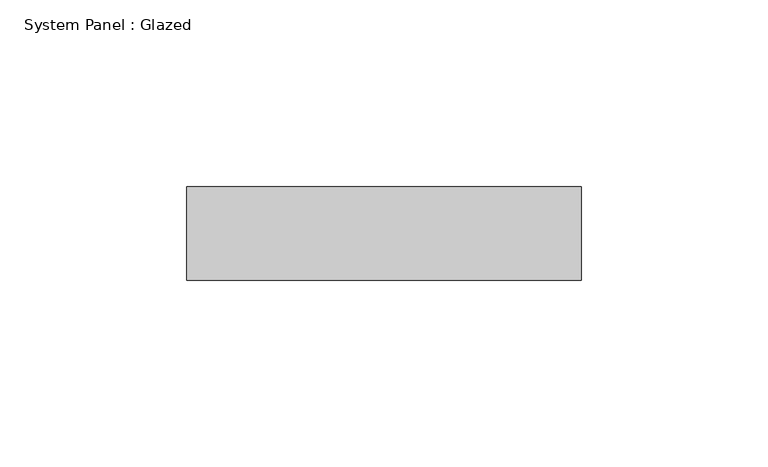
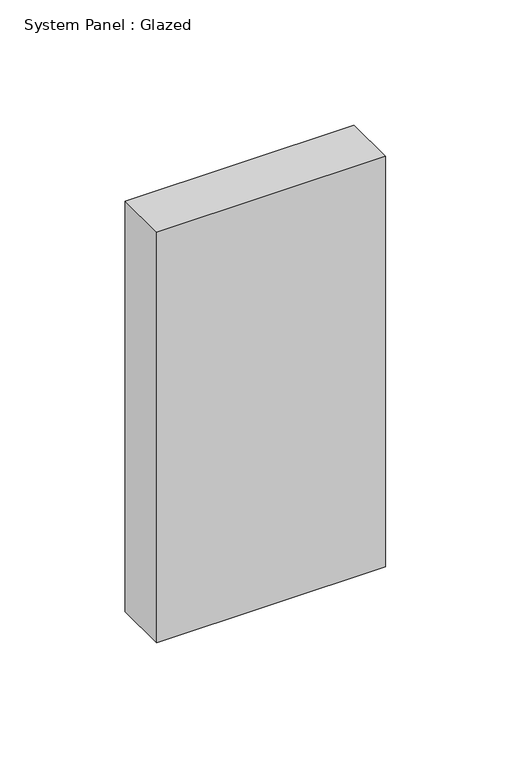
"""IFC4 building model written with IfcOpenShell, lengths in millimetres: plate geometry, System Panel : Glazed."""

from ifc_helpers import new_model, si_unit, origin, origin_with_axes, place, context, project, spatial, polyline, outline, extrude, source, transform, mapped, element, save


def system_panel_glazed_969c784e(model_context):
    return source(origin(), model_context, "Body", "SweptSolid", [
        extrude(outline(polyline([(52.8128058, 24.5), (-52.8128058, 24.5), (-52.8128058, 49.5), (52.8128058, 49.5), (52.8128058, 24.5)])), origin_with_axes(), (0.0, 0.0, 1.0), 200.0),
    ])


if __name__ == "__main__":
    model = new_model("IFC4")
    model_context = context("Model", 3, world=origin())
    ifc_project = project(units=[si_unit("LENGTHUNIT", "METRE", prefix="MILLI")], contexts=[model_context])
    site = spatial("IfcSite", under=ifc_project)
    building = spatial("IfcBuilding", under=site)
    placement = place(None, origin())
    system_panel_glazed_shape = system_panel_glazed_969c784e(model_context)
    element("IfcPlate", 1, ObjectType="System Panel : Glazed", at=placement, inside=building, context=model_context, shape_type="MappedRepresentation", body=[
        mapped(system_panel_glazed_shape, transform((0.0, 0.0, 0.0), x_axis=(1.0, 0.0, 0.0), y_axis=(0.0, 1.0, 0.0), z_axis=(0.0, 0.0, 1.0))),
    ])
    save(model, "model.ifc")

# Revit data of these elements
# Element 1 (IfcPlate, "System Panel : Glazed")
#   Materials on its faces: "Glass"
# Materials
#   "Glass": class "Glass", colour RGB 218 227 224, transparency 0.85, Description = "Soda Lime Glass", Cost = 0
